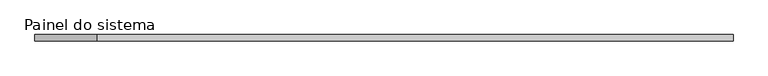
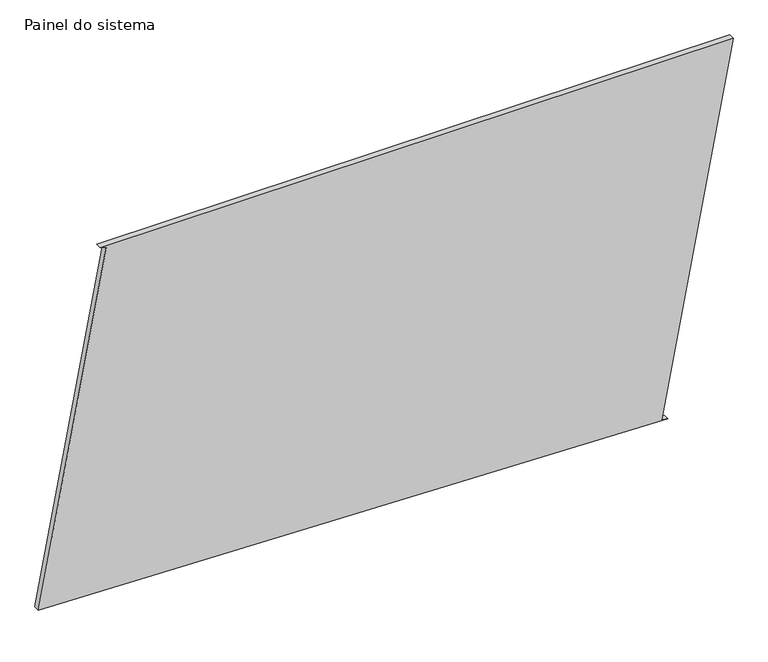
"""IFC4 building model written with IfcOpenShell, lengths in millimetres: plate geometry, Painel do sistema : Envidraçado."""

from ifc_helpers import new_model, si_unit, frame, origin, place, context, project, spatial, polyline, outline, extrude, source, transform, mapped, element, save


def painel_do_sistema_91fb9762(model_context):
    return source(origin(), model_context, "Body", "SweptSolid", [
        extrude(outline(polyline([(0.0, 1155.8024493), (4.6288169, 1131.2347052), (1553.3024618, 1423.0208244), (1553.3024618, -1169.4322305), (1548.6736449, -1144.8644863), (72.3409423, -1423.0208244), (0.0, 1155.8024493)])), frame((0.0, 24.5, 0.0), z_axis=(0.0, 1.0, 0.0), x_axis=(0.0, 0.0, 1.0)), (0.0, 0.0, 1.0), 25.0),
    ])


if __name__ == "__main__":
    model = new_model("IFC4")
    model_context = context("Model", 3, world=origin())
    ifc_project = project(units=[si_unit("LENGTHUNIT", "METRE", prefix="MILLI")], contexts=[model_context])
    site = spatial("IfcSite", under=ifc_project)
    building = spatial("IfcBuilding", under=site)
    placement = place(None, origin())
    painel_do_sistema_shape = painel_do_sistema_91fb9762(model_context)
    element("IfcPlate", 1, ObjectType="Painel do sistema : Envidraçado", at=placement, inside=building, context=model_context, shape_type="MappedRepresentation", body=[
        mapped(painel_do_sistema_shape, transform((0.0, 0.0, 0.0), x_axis=(1.0, 0.0, 0.0), y_axis=(0.0, 1.0, 0.0), z_axis=(0.0, 0.0, 1.0))),
    ])
    save(model, "model.ifc")

# Revit data of these elements
# Type "Painel do sistema : Envidraçado"
#   Construction Type Id = "GSP4R"
#   Analytic Construction = "Vidraça única Pilkington 1/8 pol"
#   Visual Light Transmittance = 0.9
#   Solar Heat Gain Coefficient = 0.86
#   Heat Transfer Coefficient (U) = 6.7069 W/(m²·K)
# Element 1 (IfcPlate, "Painel do sistema : Envidraçado")
#   Materials on its faces: "Vidro"
# Materials
#   "Vidro": class "Vidro", colour RGB 0 128 192, transparency 0.9, Description = "Vidro de sílica", Cost = 0
